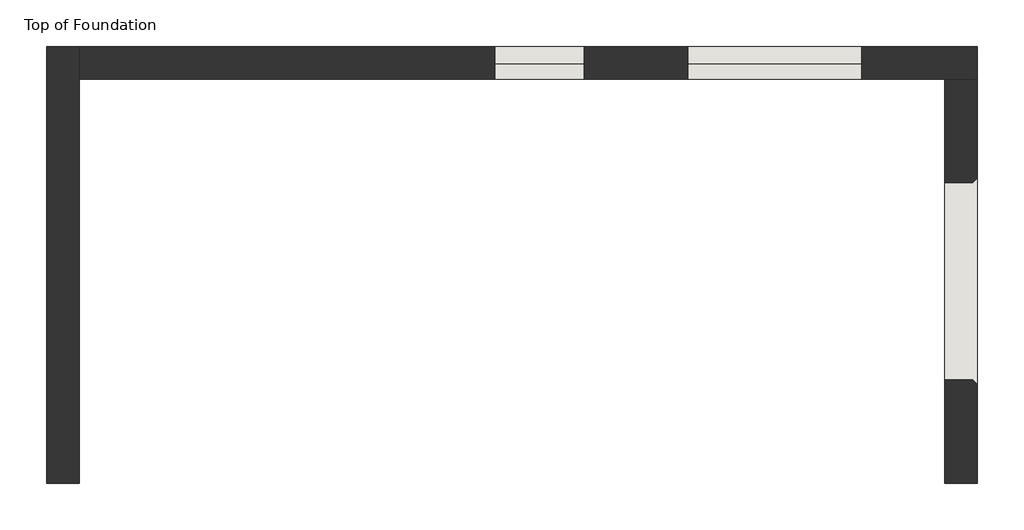
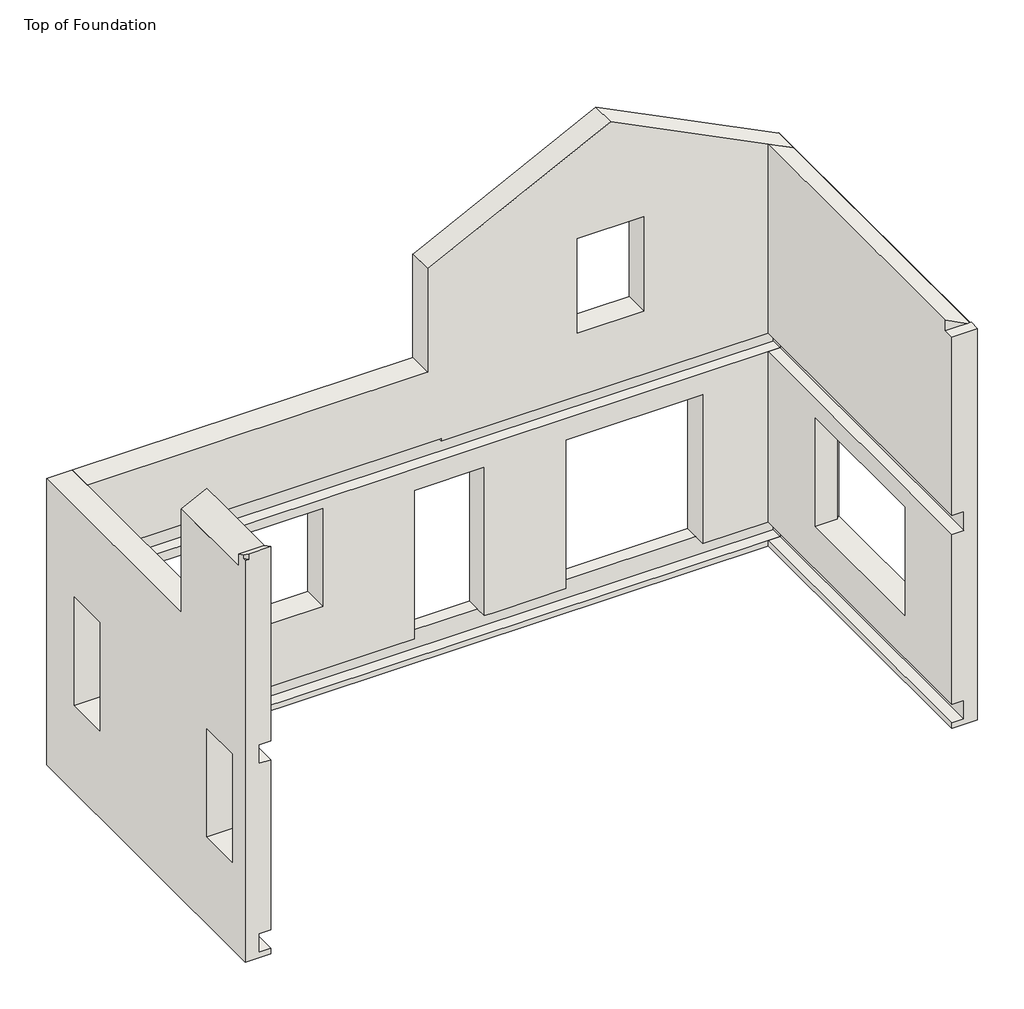
# One storey: 3 walls.
"""IFC4 building model written with IfcOpenShell, lengths in millimetres."""

import ifcopenshell
import ifcopenshell.guid

model = None  # the IFC model being written
_history = None  # IfcOwnerHistory: only IFC2X3 demands one
_inside = {}  # id of a spatial element -> (the spatial element, [elements in it])
_under = {}  # id of a project, library or spatial element -> (it, [spatial elements below it])
_declared = {}  # id of a project -> (the project, [libraries it declares])
_typed = {}  # id of a type object -> (the type object, [elements of that type])
_made_of = {}  # id of a material, layer set ... -> (it, [elements and type objects made of it])


def new_model(schema):
    """Start an empty IFC model of exactly this schema.

    Asked for "IFC4X3", IfcOpenShell would pick the latest addendum, in which some entities
    have other attributes; the version numbers below select the first issue.
    IFC2X3 requires an IfcOwnerHistory on every rooted entity: one is made here for all.
    """
    global model, _history
    if schema == "IFC4X3":
        model = ifcopenshell.file(schema_version=(4, 3, 0, 0))
    else:
        model = ifcopenshell.file(schema=schema)
    _inside.clear()
    _under.clear()
    _declared.clear()
    _typed.clear()
    _made_of.clear()
    _history = None
    if model.schema == "IFC2X3":
        org = make("IfcOrganization", Name="unknown")
        user = make(
            "IfcPersonAndOrganization",
            ThePerson=make("IfcPerson", FamilyName="unknown"),
            TheOrganization=org,
        )
        app = make(
            "IfcApplication",
            ApplicationDeveloper=org,
            Version="unknown",
            ApplicationFullName="unknown",
            ApplicationIdentifier="unknown",
        )
        _history = make(
            "IfcOwnerHistory",
            OwningUser=user,
            OwningApplication=app,
            ChangeAction="ADDED",
            CreationDate=0,
        )
    return model


def make(cls, **values):
    """One entity of the class cls with the attributes given. An attribute that is None is left unset."""
    return model.create_entity(
        cls, **{name: value for name, value in values.items() if value is not None}
    )


def rooted(cls, **values):
    """An entity with a GlobalId (a new one), such as an element, a storey or a relation."""
    return make(cls, GlobalId=ifcopenshell.guid.new(), OwnerHistory=_history, **values)


def si_unit(unit_type, name, prefix=None):
    """IfcSIUnit, for example si_unit("LENGTHUNIT", "METRE", prefix="MILLI")."""
    return make("IfcSIUnit", UnitType=unit_type, Prefix=prefix, Name=name)


def assignment(units):
    """IfcUnitAssignment: the units of a project."""
    return None if units is None else make("IfcUnitAssignment", Units=units)


def point(xyz):
    """IfcCartesianPoint."""
    return None if xyz is None else make("IfcCartesianPoint", Coordinates=xyz)


def direction(xyz):
    """IfcDirection."""
    return None if xyz is None else make("IfcDirection", DirectionRatios=xyz)


def frame(location, z_axis=None, x_axis=None):
    """IfcAxis2Placement3D, a coordinate frame: its origin and axes. An axis left out is left unset."""
    return make(
        "IfcAxis2Placement3D",
        Location=point(location),
        Axis=direction(z_axis),
        RefDirection=direction(x_axis),
    )


def origin():
    """The frame at (0, 0, 0) with its axes left unset."""
    return frame((0.0, 0.0, 0.0))


def place(relative_to, where):
    """IfcLocalPlacement: puts the frame where relative to a parent placement (None: the world)."""
    return make(
        "IfcLocalPlacement", PlacementRelTo=relative_to, RelativePlacement=where
    )


def context(
    kind, dimensions, precision=None, world=None, true_north=None, identifier=None
):
    """IfcGeometricRepresentationContext, for example the 3D "Model" context."""
    return make(
        "IfcGeometricRepresentationContext",
        ContextIdentifier=identifier,
        ContextType=kind,
        CoordinateSpaceDimension=dimensions,
        Precision=precision,
        WorldCoordinateSystem=world,
        TrueNorth=true_north,
    )


def project(units=None, contexts=None):
    """IfcProject with its units and contexts."""
    return rooted(
        "IfcProject",
        Name="project",
        RepresentationContexts=contexts,
        UnitsInContext=assignment(units),
    )


def spatial(cls, under=None, at=None, **own):
    """A site, building, storey or space (cls), placed at a placement, below another one or the project."""
    s = rooted(cls, ObjectPlacement=at, **own)
    if under is not None:
        _under.setdefault(under.id(), (under, []))[1].append(s)
    return s


def faces_of(points, faces, orient=None, outer=None):
    """IfcFace entities. A face is a list of loops; a loop is a list of indices into points, from 0.

    orient and outer hold one flag for each loop. By default every Orientation is true, the
    first loop of a face is its IfcFaceOuterBound and the others are IfcFaceBound.
    """
    made = []
    for i, loops in enumerate(faces):
        bounds = []
        for j, loop in enumerate(loops):
            is_outer = j == 0 if outer is None else outer[i][j]
            bounds.append(
                make(
                    "IfcFaceOuterBound" if is_outer else "IfcFaceBound",
                    Bound=make("IfcPolyLoop", Polygon=[points[k] for k in loop]),
                    Orientation=True if orient is None else orient[i][j],
                )
            )
        made.append(make("IfcFace", Bounds=bounds))
    return made


def faceted_brep(points, faces, orient=None, outer=None, voids=None):
    """IfcFacetedBrep: a solid bounded by flat faces; with voids (closed shells), ...WithVoids."""
    shared = [point(p) for p in points]
    hull = make("IfcClosedShell", CfsFaces=faces_of(shared, faces, orient, outer))
    if voids is None:
        return make("IfcFacetedBrep", Outer=hull)
    return make(
        "IfcFacetedBrepWithVoids",
        Outer=hull,
        Voids=[
            make(cls, CfsFaces=faces_of(shared, fs, o, b)) for cls, fs, o, b in voids
        ],
    )


def shape(context_of_items, identifier, shape_type, items):
    """IfcShapeRepresentation: the items that make up one representation, for example the "Body"."""
    return make(
        "IfcShapeRepresentation",
        ContextOfItems=context_of_items,
        RepresentationIdentifier=identifier,
        RepresentationType=shape_type,
        Items=items,
    )


def made_of(thing, what):
    """Note that an element or type object is made of a material, layer set ...; save() writes the relation."""
    if what is not None:
        _made_of.setdefault(what.id(), (what, []))[1].append(thing)
    return thing


def element(
    cls,
    number,
    at=None,
    inside=None,
    cuts=None,
    type_object=None,
    material=None,
    context=None,
    identifier="Body",
    shape_type=None,
    held_by="IfcProductDefinitionShape",
    body=None,
    shapes=None,
    **own,
):
    """One element of the class cls, such as IfcWall. Its Tag is "e" and its number.

    at: its placement. inside: the storey or other place that contains it. cuts: it is an
    opening in that element (IfcRelVoidsElement). A single representation is given by context,
    identifier, shape_type and body (its items); several are given by shapes. held_by: the class
    of the entity that holds the representations. save() writes the other relations.
    """
    e = rooted(cls, Tag="e%d" % number, ObjectPlacement=at, **own)
    if body is not None:
        shapes = [shape(context, identifier, shape_type, body)]
    if shapes is not None:
        e.Representation = make(held_by, Representations=shapes)
    if inside is not None:
        _inside.setdefault(inside.id(), (inside, []))[1].append(e)
    if cuts is not None:
        rooted(
            "IfcRelVoidsElement", RelatingBuildingElement=cuts, RelatedOpeningElement=e
        )
    if type_object is not None:
        _typed.setdefault(type_object.id(), (type_object, []))[1].append(e)
    return made_of(e, material)


def aggregate(whole, parts):
    """IfcRelAggregates: a whole, such as a stair, and the parts it consists of."""
    return rooted("IfcRelAggregates", RelatingObject=whole, RelatedObjects=parts)


def save(model, path):
    """Write the relations noted so far, then the file.

    IfcRelAggregates (storeys below a building ...), IfcRelContainedInSpatialStructure (elements
    in a storey), IfcRelDefinesByType, IfcRelAssociatesMaterial and IfcRelDeclares: one each for
    every whole, place, type object, material and project.
    """
    for whole, parts in _under.values():
        aggregate(whole, parts)
    for where, things in _inside.values():
        rooted(
            "IfcRelContainedInSpatialStructure",
            RelatedElements=things,
            RelatingStructure=where,
        )
    for kind, things in _typed.values():
        rooted("IfcRelDefinesByType", RelatedObjects=things, RelatingType=kind)
    for what, things in _made_of.values():
        rooted("IfcRelAssociatesMaterial", RelatedObjects=things, RelatingMaterial=what)
    for by, libraries in _declared.values():
        rooted("IfcRelDeclares", RelatingContext=by, RelatedDefinitions=libraries)
    model.write(path)


model = new_model("IFC4")

# Units and contexts
model_context = context("Model", 3, world=origin())
ifc_project = project(units=[si_unit("LENGTHUNIT", "METRE", prefix="MILLI")], contexts=[model_context])

# Site, building, storey
site = spatial("IfcSite", under=ifc_project)
building = spatial("IfcBuilding", under=site)
storey = spatial("IfcBuildingStorey", under=building, Name="Top of Foundation", Elevation=-349.25)

# Walls
placement = place(None, origin())
element("IfcWall", 1, ObjectType="Exterior - Brick on Mtl. Stud", at=placement, inside=storey, context=model_context, shape_type="Brep", body=[
    faceted_brep([(-5636.7553068, 3152.0888758, -349.25), (-5636.7553068, 7524.0638758, -349.25), (-5636.7553068, 7876.4888758, -349.25), (-5636.7553068, 7876.4888758, 3810.0), (-5636.7553068, 7524.0638758, 3810.0), (-5636.7553068, 4676.0888758, 3810.0), (-5636.7553068, 4676.0888758, 5486.4), (-5636.7553068, 4323.6638758, 5486.4), (-5636.7553068, 3304.4888758, 5486.4), (-5636.7553068, 3304.4888758, 5488.5342644), (-5636.7553068, 3152.0888758, 5564.7342644), (-5636.7553068, 3152.0888758, 2743.2), (-5636.7553068, 4323.6638758, 2743.2), (-5636.7553068, 4488.7638758, 2743.2), (-5636.7553068, 4488.7638758, 2781.3), (-5636.7553068, 4676.0888758, 2781.3), (-5636.7553068, 7524.0638758, 2781.3), (-5636.7553068, 7689.1638758, 2781.3), (-5636.7553068, 7689.1638758, 2470.15), (-5636.7553068, 7524.0638758, 2470.15), (-5636.7553068, 7219.2638758, 2470.15), (-5636.7553068, 7219.2638758, 914.4), (-5636.7553068, 6609.6638758, 914.4), (-5636.7553068, 6609.6638758, 2470.15), (-5636.7553068, 4066.4888758, 2470.15), (-5636.7553068, 4066.4888758, 914.4), (-5636.7553068, 3456.8888758, 914.4), (-5636.7553068, 3456.8888758, 2470.15), (-5636.7553068, 3152.0888758, 2470.15), (-5636.7553068, 3152.0888758, 0.0), (-5636.7553068, 7524.0638758, 0.0), (-5636.7553068, 7689.1638758, 0.0), (-5636.7553068, 7689.1638758, -273.05), (-5636.7553068, 7524.0638758, -273.05), (-5636.7553068, 3152.0888758, -273.05), (-5989.1803068, 7876.4888758, -349.25), (-5989.1803068, 3152.0888758, -349.25), (-5989.1803068, 3152.0888758, 5486.4), (-5989.1803068, 3199.7138758, 5486.4), (-5989.1803068, 3199.7138758, 5540.9217644), (-5989.1803068, 3304.4888758, 5488.5342644), (-5989.1803068, 3304.4888758, 5312.3217644), (-5989.1803068, 4676.0888758, 5312.3217644), (-5989.1803068, 4676.0888758, 3810.0), (-5989.1803068, 7876.4888758, 3810.0), (-5989.1803068, 3456.8888758, 2489.2), (-5989.1803068, 3456.8888758, 914.4), (-5989.1803068, 4066.4888758, 914.4), (-5989.1803068, 4066.4888758, 2489.2), (-5989.1803068, 6609.6638758, 2489.2), (-5989.1803068, 6609.6638758, 914.4), (-5989.1803068, 7219.2638758, 914.4), (-5989.1803068, 7219.2638758, 2489.2), (-5801.8553068, 3152.0888758, -273.05), (-5801.8553068, 3152.0888758, 0.0), (-5801.8553068, 3152.0888758, 2470.15), (-5801.8553068, 3152.0888758, 2743.2), (-5941.5553068, 3152.0888758, 5564.7342644), (-5941.5553068, 3152.0888758, 5486.4), (-5984.911778, 4676.0888758, 5312.3217644), (-5937.286778, 3304.4888758, 5336.1342644), (-5984.911778, 3304.4888758, 5312.3217644), (-5801.8553068, 3456.8888758, 2489.2), (-5801.8553068, 3456.8888758, 2470.15), (-5801.8553068, 4066.4888758, 2470.15), (-5801.8553068, 4066.4888758, 2489.2), (-5801.8553068, 6609.6638758, 2489.2), (-5801.8553068, 6609.6638758, 2470.15), (-5801.8553068, 7219.2638758, 2470.15), (-5801.8553068, 7219.2638758, 2489.2), (-5801.8553068, 7689.1638758, -273.05), (-5801.8553068, 7689.1638758, 0.0), (-5801.8553068, 7689.1638758, 2470.15), (-5801.8553068, 4488.7638758, 2470.15), (-5801.8553068, 4488.7638758, 2743.2), (-5801.8553068, 7689.1638758, 2781.3), (-5801.8553068, 4488.7638758, 2781.3)], [[[0, 1, 2, 3, 4, 5, 6, 7, 8, 9, 10, 11, 12, 13, 14, 15, 16, 17, 18, 19, 20, 21, 22, 23, 24, 25, 26, 27, 28, 29, 30, 31, 32, 33, 34]], [[35, 36, 37, 38, 39, 40, 41, 42, 43, 44], [45, 46, 47, 48], [49, 50, 51, 52]], [[2, 1, 0, 36, 35]], [[5, 4, 3, 44, 43]], [[37, 36, 0, 34, 53, 54, 29, 28, 55, 56, 11, 10, 57, 58]], [[3, 2, 35, 44]], [[6, 5, 43, 42, 59]], [[41, 40, 9, 8, 60, 61]], [[38, 37, 58]], [[38, 58, 57, 39]], [[8, 7, 6, 59, 61, 60]], [[42, 41, 61, 59]], [[10, 9, 40, 39, 57]], [[46, 45, 62, 63, 27, 26]], [[47, 46, 26, 25]], [[48, 47, 25, 24, 64, 65]], [[45, 48, 65, 62]], [[50, 49, 66, 67, 23, 22]], [[51, 50, 22, 21]], [[52, 51, 21, 20, 68, 69]], [[49, 52, 69, 66]], [[70, 53, 34, 33, 32]], [[71, 31, 30, 29, 54]], [[71, 70, 32, 31]], [[70, 71, 54, 53]], [[72, 68, 20, 19, 18]], [[64, 24, 23, 67, 73]], [[63, 55, 28, 27]], [[56, 74, 13, 12, 11]], [[55, 63, 62, 65, 64, 73, 67, 66, 69, 68, 72, 75, 76, 74, 56]], [[76, 75, 17, 16, 15, 14]], [[75, 72, 18, 17]], [[74, 76, 14, 13]]]),
])
element("IfcWall", 2, ObjectType="Exterior - Brick on Mtl. Stud", at=placement, inside=storey, context=model_context, shape_type="Brep", body=[
    faceted_brep([(-5636.7553068, 7524.0638758, -349.25), (3716.7946932, 7524.0638758, -349.25), (4069.2196932, 7524.0638758, -349.25), (4069.2196932, 7524.0638758, 5312.3217644), (4064.9511643, 7524.0638758, 5312.3217644), (3716.7946932, 7524.0638758, 5486.4), (1554.6196932, 7524.0638758, 6567.4875), (-607.5553068, 7524.0638758, 5486.4), (-955.711778, 7524.0638758, 5312.3217644), (-959.9803068, 7524.0638758, 5312.3217644), (-959.9803068, 7524.0638758, 3810.0), (-5636.7553068, 7524.0638758, 3810.0), (-5636.7553068, 7524.0638758, 2781.3), (-959.9803068, 7524.0638758, 2781.3), (-772.6553068, 7524.0638758, 2781.3), (-772.6553068, 7524.0638758, 2743.2), (-607.5553068, 7524.0638758, 2743.2), (3716.7946932, 7524.0638758, 2743.2), (3881.8946932, 7524.0638758, 2743.2), (3881.8946932, 7524.0638758, 2470.15), (3716.7946932, 7524.0638758, 2470.15), (43.3196932, 7524.0638758, 2470.15), (-77.3303068, 7524.0638758, 2470.15), (-1480.6803068, 7524.0638758, 2470.15), (-1601.3303068, 7524.0638758, 2470.15), (-5636.7553068, 7524.0638758, 2470.15), (-5636.7553068, 7524.0638758, 0.0), (-1601.3303068, 7524.0638758, 0.0), (-1480.6803068, 7524.0638758, 0.0), (-1144.1303068, 7524.0638758, 0.0), (-1144.1303068, 7524.0638758, 2159.0), (-178.9303068, 7524.0638758, 2159.0), (-178.9303068, 7524.0638758, 0.0), (-77.3303068, 7524.0638758, 0.0), (43.3196932, 7524.0638758, 0.0), (940.2571932, 7524.0638758, 0.0), (940.2571932, 7524.0638758, 2159.0), (2819.8571932, 7524.0638758, 2159.0), (2819.8571932, 7524.0638758, 0.0), (3716.7946932, 7524.0638758, 0.0), (3881.8946932, 7524.0638758, 0.0), (3881.8946932, 7524.0638758, -273.05), (3716.7946932, 7524.0638758, -273.05), (-5636.7553068, 7524.0638758, -273.05), (1097.4196932, 7524.0638758, 3657.6), (1097.4196932, 7524.0638758, 5029.2), (2011.8196932, 7524.0638758, 5029.2), (2011.8196932, 7524.0638758, 3657.6), (-2399.8428068, 7524.0638758, 2336.8), (-2399.8428068, 7524.0638758, 914.4), (-4838.2428068, 7524.0638758, 914.4), (-4838.2428068, 7524.0638758, 2336.8), (4069.2196932, 7876.4888758, -349.25), (-5636.7553068, 7876.4888758, -349.25), (-5636.7553068, 7876.4888758, 3810.0), (-959.9803068, 7876.4888758, 3810.0), (-959.9803068, 7876.4888758, 5312.3217644), (-955.711778, 7876.4888758, 5312.3217644), (1554.6196932, 7876.4888758, 6567.4875), (4064.9511643, 7876.4888758, 5312.3217644), (4069.2196932, 7876.4888758, 5312.3217644), (1097.4196932, 7876.4888758, 5029.2), (1097.4196932, 7876.4888758, 3657.6), (2011.8196932, 7876.4888758, 3657.6), (2011.8196932, 7876.4888758, 5029.2), (-1144.1303068, 7876.4888758, 2159.0), (-1144.1303068, 7876.4888758, 0.0), (-178.9303068, 7876.4888758, 0.0), (-178.9303068, 7876.4888758, 2159.0), (-2399.8428068, 7876.4888758, 914.4), (-2399.8428068, 7876.4888758, 2336.8), (-4838.2428068, 7876.4888758, 2336.8), (-4838.2428068, 7876.4888758, 914.4), (2819.8571932, 7876.4888758, 0.0), (2819.8571932, 7876.4888758, 2159.0), (940.2571932, 7876.4888758, 2159.0), (940.2571932, 7876.4888758, 0.0), (-5636.7553068, 7689.1638758, -273.05), (-5636.7553068, 7689.1638758, 0.0), (-5636.7553068, 7689.1638758, 2470.15), (-5636.7553068, 7689.1638758, 2781.3), (4069.2196932, 7571.6888758, -349.25), (-1144.1303068, 7689.1638758, 0.0), (-178.9303068, 7689.1638758, 0.0), (2819.8571932, 7689.1638758, 0.0), (940.2571932, 7689.1638758, 0.0), (3881.8946932, 7689.1638758, -273.05), (3881.8946932, 7689.1638758, 0.0), (3881.8946932, 7689.1638758, 2470.15), (-772.6553068, 7689.1638758, 2470.15), (-772.6553068, 7689.1638758, 2743.2), (3881.8946932, 7689.1638758, 2743.2), (-772.6553068, 7689.1638758, 2781.3)], [[[0, 1, 2, 3, 4, 5, 6, 7, 8, 9, 10, 11, 12, 13, 14, 15, 16, 17, 18, 19, 20, 21, 22, 23, 24, 25, 26, 27, 28, 29, 30, 31, 32, 33, 34, 35, 36, 37, 38, 39, 40, 41, 42, 43], [44, 45, 46, 47], [48, 49, 50, 51]], [[52, 53, 54, 55, 56, 57, 58, 59, 60], [61, 62, 63, 64], [65, 66, 67, 68], [69, 70, 71, 72], [73, 74, 75, 76]], [[54, 53, 0, 43, 77, 78, 26, 25, 79, 80, 12, 11]], [[3, 2, 81, 52, 60]], [[2, 1, 0, 53, 52, 81]], [[11, 10, 55, 54]], [[10, 9, 56, 55]], [[56, 9, 8, 57]], [[8, 7, 6, 58, 57]], [[6, 5, 4, 59, 58]], [[3, 60, 59, 4]], [[62, 61, 45, 44]], [[63, 62, 44, 47]], [[64, 63, 47, 46]], [[61, 64, 46, 45]], [[30, 29, 82, 66, 65]], [[31, 30, 65, 68]], [[32, 31, 68, 67, 83]], [[67, 66, 82, 83]], [[49, 69, 72, 50]], [[70, 48, 51, 71]], [[48, 70, 69, 49]], [[50, 72, 71, 51]], [[74, 73, 84, 38, 37]], [[75, 74, 37, 36]], [[76, 75, 36, 35, 85]], [[73, 76, 85, 84]], [[41, 86, 77, 43, 42]], [[84, 87, 40, 39, 38]], [[83, 85, 35, 34, 33, 32]], [[78, 82, 29, 28, 27, 26]], [[86, 87, 84, 85, 83, 82, 78, 77]], [[87, 86, 41, 40]], [[79, 25, 24, 23, 22, 21, 20, 19, 88, 89]], [[90, 91, 18, 17, 16, 15]], [[79, 89, 88, 91, 90, 92, 80]], [[91, 88, 19, 18]], [[80, 92, 14, 13, 12]], [[92, 90, 15, 14]]]),
])
element("IfcWall", 3, ObjectType="Exterior - Brick on Mtl. Stud", at=placement, inside=storey, context=model_context, shape_type="Brep", body=[
    faceted_brep([(3716.7946932, 7524.0638758, -349.25), (3716.7946932, 3152.0888758, -349.25), (3716.7946932, 3152.0888758, -273.05), (3716.7946932, 7524.0638758, -273.05), (3716.7946932, 3304.4888758, 5336.1342644), (3716.7946932, 3304.4888758, 5486.4), (3716.7946932, 3844.2388758, 5486.4), (3716.7946932, 3964.8888758, 5486.4), (3716.7946932, 7524.0638758, 5486.4), (3716.7946932, 7524.0638758, 2743.2), (3716.7946932, 3964.8888758, 2743.2), (3716.7946932, 3844.2388758, 2743.2), (3716.7946932, 3152.0888758, 2743.2), (3716.7946932, 3152.0888758, 5336.1342644), (3716.7946932, 7524.0638758, 0.0), (3716.7946932, 3152.0888758, 0.0), (3716.7946932, 3152.0888758, 2470.15), (3716.7946932, 7524.0638758, 2470.15), (3716.7946932, 6404.8763758, 2184.4), (3716.7946932, 4271.2763758, 2184.4), (3716.7946932, 4271.2763758, 609.6), (3716.7946932, 6404.8763758, 609.6), (4069.2196932, 3152.0888758, -349.25), (4069.2196932, 7524.0638758, -349.25), (4069.2196932, 7524.0638758, 5312.3217644), (4069.2196932, 3304.4888758, 5312.3217644), (4069.2196932, 3304.4888758, 5336.1342644), (4069.2196932, 3152.0888758, 5336.1342644), (4069.2196932, 4221.8849671, 2184.4), (4069.2196932, 6454.2677845, 2184.4), (4069.2196932, 6454.2677845, 609.6), (4069.2196932, 4221.8849671, 609.6), (3881.8946932, 3152.0888758, 2743.2), (3881.8946932, 3152.0888758, 2470.15), (3881.8946932, 3152.0888758, 0.0), (3881.8946932, 3152.0888758, -273.05), (3881.8946932, 7524.0638758, -273.05), (3881.8946932, 7524.0638758, 0.0), (3881.8946932, 7524.0638758, 2470.15), (3881.8946932, 7524.0638758, 2743.2), (4064.9511643, 7524.0638758, 5312.3217644), (4064.9511643, 3304.4888758, 5312.3217644), (4017.3261643, 3304.4888758, 5336.1342644), (4019.8282845, 6404.8763758, 2184.4), (4019.8282845, 4271.2763758, 2184.4), (4019.8282845, 6404.8763758, 609.6), (4019.8282845, 4271.2763758, 609.6)], [[[0, 1, 2, 3]], [[4, 5, 6, 7, 8, 9, 10, 11, 12, 13]], [[14, 15, 16, 17], [18, 19, 20, 21]], [[22, 23, 24, 25, 26, 27], [28, 29, 30, 31]], [[1, 0, 23, 22]], [[22, 27, 13, 12, 32, 33, 16, 15, 34, 35, 2, 1]], [[24, 23, 0, 3, 36, 37, 14, 17, 38, 39, 9, 8, 40]], [[26, 25, 41, 42]], [[4, 13, 27, 26, 42]], [[8, 7, 6, 5, 42, 41, 40]], [[25, 24, 40, 41]], [[5, 4, 42]], [[43, 29, 28, 44, 19, 18]], [[45, 21, 20, 46, 31, 30]], [[43, 18, 21, 45]], [[19, 44, 46, 20]], [[44, 28, 31, 46]], [[29, 43, 45, 30]], [[35, 36, 3, 2]], [[37, 34, 15, 14]], [[36, 35, 34, 37]], [[33, 38, 17, 16]], [[39, 32, 12, 11, 10, 9]], [[38, 33, 32, 39]]]),
])

save(model, "model.ifc")

# Revit data of these elements
# Type "Exterior - Brick on Mtl. Stud"
#   Assembly Code = "B2010158"
#   Layers, outside or top first: 0' - 3 5/8" "Brick, Common" (function 4); 0' - 3" "Air" (function 3); 0' - 0" "Air Infiltration Barrier" (function 100); 0' - 0 3/4" "Plywood, Sheathing" (function 2); 0' - 6" "Metal Stud Layer" (function 1); 0' - 0" "Vapor Retarder" (function 100); 0' - 0 1/2" "Gypsum Wall Board" (function 5)
# Elements 1, 2 (IfcWall, "Exterior - Brick on Mtl. Stud")
#   Top Offset = 0' - 0"
#   Base Offset = 0' - 0"
#   wall height = 19' - 1 3/4"
#   Phase Created = New Construction
#   Base Constraint = Top of Foundation
#   Top Constraint = Roof
#   Materials on its faces: "Default Wall", "Brick, Common", "Gypsum Wall Board"
# Element 3 (IfcWall, "Exterior - Brick on Mtl. Stud")
#   Top Offset = 0' - 0"
#   Base Offset = 0' - 0"
#   wall height = 19' - 1 3/4"
#   Phase Created = New Construction
#   Base Constraint = Top of Foundation
#   Top Constraint = Roof
#   Materials on its faces: "Default Wall", "Gypsum Wall Board", "Brick, Common"
# Materials
#   "Brick, Common": class "Masonry", colour RGB 170 98 104, transparency 0, Description = "Common brick", Cost = 0
#   "Air": class "Gas", colour RGB 255 255 255, transparency 0, Description = "Air", Cost = 0
#   "Air Infiltration Barrier": class "Generic", colour RGB 127 127 127, transparency 0, Description = "physical material", Cost = 0
#   "Plywood, Sheathing": class "Wood", colour RGB 193 140 64, transparency 0, Description = "Plywood, sheathing grade", Cost = 0
#   "Metal Stud Layer": class "Metal", colour RGB 199 199 199, transparency 0, Description = "Light gauge steel framing, thermal air layer", Cost = 0
#   "Vapor Retarder": class "Generic", colour RGB 127 127 127, transparency 0, Description = "Polyethylene film membrane", Cost = 0
#   "Gypsum Wall Board": class "Generic", colour RGB 127 127 127, transparency 0, Description = "Gypsum Wall Board", Cost = 0
#   "Default Wall": class "Miscellaneous", colour RGB 128 128 128, transparency 0, Cost = 0
